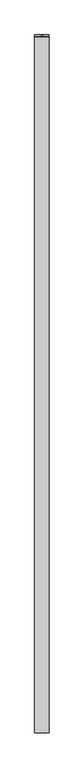
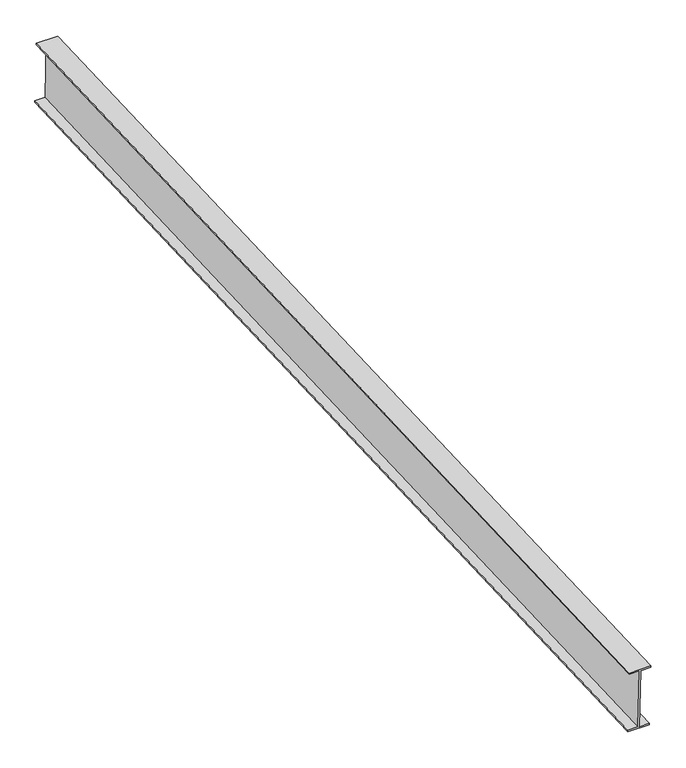
"""IFC4 building model written with IfcOpenShell, lengths in millimetres: proxy geometry, Generic Models 7:Generic Models 1:1:Generic Models 1:1 : Generic Models 7:Generic Models 1:337419:21 : Generic Models 7:Generic Models 1:1:Generic Models 1:1 : Generic Models 7:Generic Models 1:337419:306201."""

from ifc_helpers import new_model, si_unit, frame, origin, place, context, project, spatial, polyline, outline, extrude, source, transform, mapped, element, save


def generic_models_3e432a6c(model_context):
    return source(origin(), model_context, "Body", "SweptSolid", [
        extrude(outline(polyline([(126.873, 0.0), (126.873, -6.3500001), (78.994, -6.3500001), (78.994, -295.0294372), (126.873, -295.0294372), (126.873, -301.3794372), (25.527, -301.3794372), (25.527, -295.0294372), (73.406, -295.0294372), (73.406, -6.3500001), (25.527, -6.3500001), (25.527, 0.0), (126.873, 0.0)])), frame((579256.911724, -578815.1475699, 3695.4094554), z_axis=(0.0, 0.9991330730920968, 0.041630544718308224), x_axis=(-1.0, 0.0, 0.0)), (0.0, 0.0, 1.0), 4876.8),
    ])


if __name__ == "__main__":
    model = new_model("IFC4")
    model_context = context("Model", 3, world=origin())
    ifc_project = project(units=[si_unit("LENGTHUNIT", "METRE", prefix="MILLI")], contexts=[model_context])
    site = spatial("IfcSite", under=ifc_project)
    building = spatial("IfcBuilding", under=site)
    placement = place(None, origin())
    generic_models_shape = generic_models_3e432a6c(model_context)
    element("IfcBuildingElementProxy", 1, Name="Generic Models 7:Generic Models 1:1:Generic Models 1:1 : Generic Models 7:Generic Models 1:337419:21 : Generic Models 7:Generic Models 1:1:Generic Models 1:1 : Generic Models 7:Generic Models 1:337419:306201", ObjectType="Generic Models 7:Generic Models 1:1:Generic Models 1:1 : Generic Models 7:Generic Models 1:337419:21 : Generic Models 7:Generic Models 1:1:Generic Models 1:1 : Generic Models 7:Generic Models 1:337419:306201", at=placement, inside=building, context=model_context, shape_type="MappedRepresentation", body=[
        mapped(generic_models_shape, transform((0.0, 0.0, 0.0), x_axis=(1.0, 0.0, 0.0), y_axis=(0.0, 1.0, 0.0), z_axis=(0.0, 0.0, 1.0))),
    ])
    save(model, "model.ifc")

# Revit data of these elements
# Type "Generic Models 7:Generic Models 1:1:Generic Models 1:1 : Generic Models 7:Generic Models 1:337419:21 : Generic Models 7:Generic Models 1:1:Generic Models 1:1 : Generic Models 7:Generic Models 1:337419:306201"
#   NameOverride = "Generic Models 7:Generic Models 1:1:Generic Models 1:1 : Generic Models 7:Generic Models 1:337419:306201"
#   ObjectTypeOverride = "Generic Models 1:1 : Generic Models 7:Generic Models 1:337419"
#   Reference = "Generic Models 1"
#   Tag = "306201"
# Element 1 (IfcBuildingElementProxy, "Generic Models 7:Generic Models 1:1:Generic Models 1:1 : Generic Models 7:Generic Models 1:337419:21 : Generic Models 7:Generic Models 1:1:Generic Models 1:1 : Generic Models 7:Generic Models 1:337419:306201")
#   Materials on its faces: "'ZEE' SECTION (8.0x3.5Z - SEE STRUCT. DWGS)"
# Materials
#   "'ZEE' SECTION (8.0x3.5Z - SEE STRUCT. DWGS)": class "Unassigned", colour RGB 210 209 208, transparency 0, Keynote = "M05121300.02", Cost = 0
